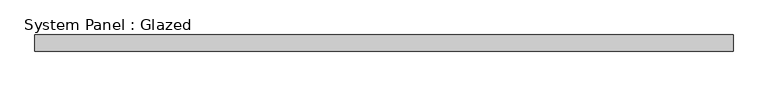
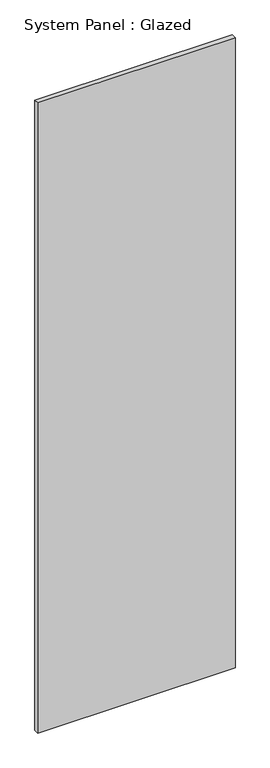
"""IFC4 building model written with IfcOpenShell, lengths in millimetres: plate geometry, System Panel : Glazed."""

from ifc_helpers import new_model, si_unit, origin, origin_with_axes, place, context, project, spatial, polyline, outline, extrude, source, transform, mapped, element, save


def system_panel_glazed_44e43824(model_context):
    return source(origin(), model_context, "Body", "SweptSolid", [
        extrude(outline(polyline([(542.0483058, -44.45), (-542.0483058, -44.45), (-542.0483058, -19.05), (542.0483058, -19.05), (542.0483058, -44.45)])), origin_with_axes(), (0.0, 0.0, 1.0), 3657.6),
    ])


if __name__ == "__main__":
    model = new_model("IFC4")
    model_context = context("Model", 3, world=origin())
    ifc_project = project(units=[si_unit("LENGTHUNIT", "METRE", prefix="MILLI")], contexts=[model_context])
    site = spatial("IfcSite", under=ifc_project)
    building = spatial("IfcBuilding", under=site)
    placement = place(None, origin())
    system_panel_glazed_shape = system_panel_glazed_44e43824(model_context)
    element("IfcPlate", 1, ObjectType="System Panel : Glazed", at=placement, inside=building, context=model_context, shape_type="MappedRepresentation", body=[
        mapped(system_panel_glazed_shape, transform((0.0, 0.0, 0.0), x_axis=(1.0, 0.0, 0.0), y_axis=(0.0, 1.0, 0.0), z_axis=(0.0, 0.0, 1.0))),
    ])
    save(model, "model.ifc")

# Revit data of these elements
# Type "System Panel : Glazed"
#   Construction Type Id = "GSP4R"
#   Analytic Construction = "1/8 in Pilkington single glazing"
#   Visual Light Transmittance = 0.9
#   Solar Heat Gain Coefficient = 0.86
#   Heat Transfer Coefficient (U) = 1.18115 BTU/(h·ft²·°F)
#   Define Thermal Properties by = 1
# Element 1 (IfcPlate, "System Panel : Glazed")
#   Materials on its faces: "Glass"
# Materials
#   "Glass": class "Glass", colour RGB 0 128 192, transparency 0.75, Description = "Soda Lime Glass", Cost = 0
